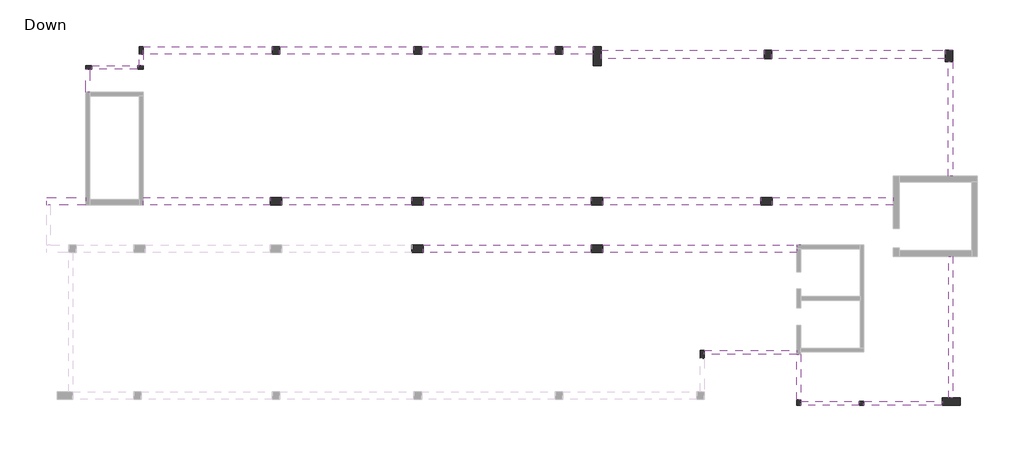
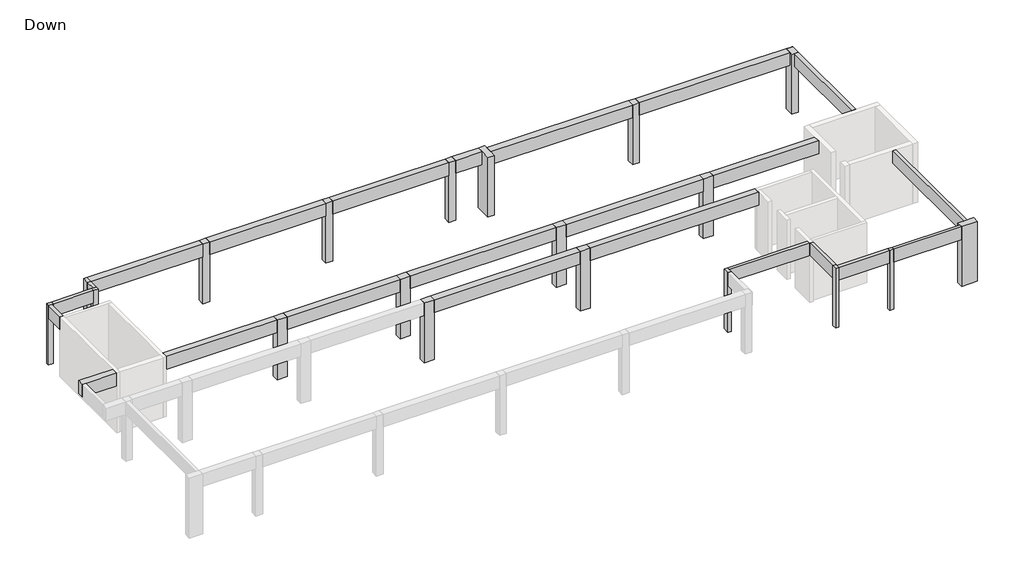
# One storey, part 2 of 2: 23 beams, 19 columns.
"""IFC4 building model written with IfcOpenShell, lengths in millimetres."""

from ifc_helpers import new_model, si_unit, frame, origin, origin_with_axes, place, context, project, spatial, polyline, outline, extrude, faceted_brep, element, save

model = new_model("IFC4")

# Units and contexts
model_context = context("Model", 3, world=origin())
ifc_project = project(units=[si_unit("LENGTHUNIT", "METRE", prefix="MILLI")], contexts=[model_context])

# Site, building, storey
site = spatial("IfcSite", under=ifc_project)
building = spatial("IfcBuilding", under=site)
storey = spatial("IfcBuildingStorey", under=building, Name="Down", Elevation=0.0)

# Beams
placement = place(None, origin())
element("IfcBeam", 1, ObjectType="Concrete Rectengular Beam : 20/80", at=placement, inside=storey, context=model_context, shape_type="Brep", body=[
    faceted_brep([(-14307.5920656, 7355.2095413, 3800.0), (-14307.5920656, 7555.2095413, 3800.0), (-16709.1027603, 7555.2095413, 3800.0), (-16709.1027603, 7355.2095413, 3800.0), (-16709.1027603, 7355.2095413, 3520.0), (-16709.1027603, 7355.2095413, 3000.0), (-14307.5920656, 7355.2095413, 3000.0), (-14307.5920656, 7355.2095413, 3520.0), (-14307.5920656, 7555.2095413, 3000.0), (-16709.1027603, 7555.2095413, 3000.0)], [[[0, 1, 2, 3]], [[0, 3, 4, 5, 6, 7]], [[8, 6, 5, 9]], [[1, 8, 9, 2]], [[1, 0, 7, 6, 8]], [[3, 2, 9, 5, 4]]]),
])
element("IfcBeam", 2, ObjectType="Concrete Rectengular Beam : 20/80", at=placement, inside=storey, context=model_context, shape_type="Brep", body=[
    faceted_brep([(-16809.1027603, 7355.2095413, 3800.0), (-17009.1027603, 7355.2095413, 3800.0), (-17009.1027603, 6157.8562202, 3800.0), (-16809.1027603, 6157.8562202, 3800.0), (-17009.1027603, 7355.2095413, 3000.0), (-17009.1027603, 6157.8562202, 3000.0), (-16809.1027603, 7355.2095413, 3000.0), (-16809.1027603, 6157.8562202, 3000.0), (-16809.1027603, 7355.2095413, 3520.0), (-16809.1027603, 6157.8562202, 3520.0)], [[[0, 1, 2, 3]], [[1, 4, 5, 2]], [[4, 6, 7, 5]], [[6, 8, 0, 3, 9, 7]], [[0, 8, 6, 4, 1]], [[3, 2, 5, 7, 9]]]),
])
element("IfcBeam", 3, ObjectType="Concrete Rectengular Beam : 20/80", at=placement, inside=storey, context=model_context, shape_type="Brep", body=[
    faceted_brep([(28136.856558, -9844.9662281, 3800.0), (28336.856558, -9844.9662281, 3800.0), (28336.856558, -2441.3717827, 3800.0), (28136.856558, -2441.3717827, 3800.0), (28336.856558, -9844.9662281, 3000.0), (28336.856558, -2441.3717827, 3000.0), (28136.856558, -9844.9662281, 3000.0), (28136.856558, -2441.3717827, 3000.0), (28136.856558, -9844.9662281, 3520.0), (28136.856558, -2441.3717827, 3520.0)], [[[0, 1, 2, 3]], [[1, 4, 5, 2]], [[4, 6, 7, 5]], [[6, 8, 0, 3, 9, 7]], [[1, 0, 8, 6, 4]], [[3, 2, 5, 7, 9]]]),
])
element("IfcBeam", 4, ObjectType="Concrete Rectengular Beam : 20/80", at=placement, inside=storey, context=model_context, shape_type="Brep", body=[
    faceted_brep([(23695.2926489, -10044.9662281, 3800.0), (23695.2926489, -10244.9662281, 3800.0), (27784.8345171, -10244.9662281, 3800.0), (27784.8345171, -10044.9662281, 3800.0), (23695.2926489, -10244.9662281, 3000.0), (27784.8345171, -10244.9662281, 3000.0), (23695.2926489, -10044.9662281, 3000.0), (27784.8345171, -10044.9662281, 3000.0), (27784.8345171, -10044.9662281, 3520.0)], [[[0, 1, 2, 3]], [[1, 4, 5, 2]], [[4, 6, 7, 5]], [[6, 0, 3, 8, 7]], [[1, 0, 6, 4]], [[3, 2, 5, 7, 8]]]),
])
element("IfcBeam", 5, ObjectType="Concrete Rectengular Beam : 20/80", at=placement, inside=storey, context=model_context, shape_type="Brep", body=[
    faceted_brep([(20395.2300261, -10044.9662281, 3800.0), (20395.2300261, -10244.9662281, 3800.0), (23445.2926489, -10244.9662281, 3800.0), (23445.2926489, -10044.9662281, 3800.0), (20395.2300261, -10044.9662281, 3000.0), (20395.2300261, -10044.9662281, 3520.0), (23445.2926489, -10044.9662281, 3000.0), (20395.2300261, -10244.9662281, 3000.0), (23445.2926489, -10244.9662281, 3000.0)], [[[0, 1, 2, 3]], [[4, 5, 0, 3, 6]], [[7, 4, 6, 8]], [[1, 7, 8, 2]], [[1, 0, 5, 4, 7]], [[3, 2, 8, 6]]]),
])
element("IfcBeam", 6, ObjectType="Concrete Rectengular Beam : 20/80", at=placement, inside=storey, context=model_context, shape_type="SweptSolid", body=[
    extrude(outline(polyline([(20195.2300261, -7584.1322554), (20395.2300261, -7584.1322554), (20395.2300261, -9947.194205), (20195.2300261, -9947.194205), (20195.2300261, -7584.1322554)])), frame((0.0, 0.0, 3000.0), z_axis=(0.0, 0.0, 1.0), x_axis=(1.0, 0.0, 0.0)), (0.0, 0.0, 1.0), 800.0),
])
element("IfcBeam", 7, ObjectType="Concrete Rectengular Beam : 20/80", at=placement, inside=storey, context=model_context, shape_type="Brep", body=[
    faceted_brep([(15344.7363769, -7371.4322554, 3800.0), (15344.7363769, -7571.4322554, 3800.0), (20195.2300261, -7571.4322554, 3800.0), (20195.2300261, -7371.4322554, 3800.0), (20195.2300261, -7371.4322554, 3520.0), (20195.2300261, -7371.4322554, 3000.0), (15344.7363769, -7371.4322554, 3000.0), (15344.7363769, -7371.4322554, 3520.0), (15344.7363769, -7571.4322554, 3000.0), (20195.2300261, -7571.4322554, 3000.0)], [[[0, 1, 2, 3]], [[0, 3, 4, 5, 6, 7]], [[8, 6, 5, 9]], [[1, 8, 9, 2]], [[1, 0, 7, 6, 8]], [[3, 2, 9, 5, 4]]]),
])
element("IfcBeam", 8, ObjectType="Concrete Rectengular Beam : 20/80", at=placement, inside=storey, context=model_context, shape_type="Brep", body=[
    faceted_brep([(-14207.5920656, 7555.2095413, 3800.0), (-14007.5920656, 7555.2095413, 3800.0), (-14007.5920656, 8151.3324092, 3800.0), (-14207.5920656, 8151.3324092, 3800.0), (-14207.5920656, 7555.2095413, 3000.0), (-14207.5920656, 8151.3324092, 3000.0), (-14007.5920656, 7555.2095413, 3000.0), (-14007.5920656, 8151.3324092, 3000.0), (-14007.5920656, 7555.2095413, 3520.0), (-14007.5920656, 8151.3324092, 3520.0)], [[[0, 1, 2, 3]], [[4, 0, 3, 5]], [[6, 4, 5, 7]], [[2, 1, 8, 6, 7, 9]], [[0, 4, 6, 8, 1]], [[5, 3, 2, 9, 7]]]),
])
element("IfcBeam", 9, ObjectType="Concrete Rectengular Beam : 25/80", at=placement, inside=storey, context=model_context, shape_type="Brep", body=[
    faceted_brep([(28351.2236194, 7751.6453791, 3800.0), (28101.2236194, 7751.6453791, 3800.0), (28101.2236194, 1758.6282173, 3800.0), (28351.2236194, 1758.6282173, 3800.0), (28101.2236194, 7751.6453791, 3520.0), (28101.2236194, 7751.6453791, 3000.0), (28101.2236194, 1758.6282173, 3000.0), (28101.2236194, 1758.6282173, 3520.0), (28351.2236194, 7751.6453791, 3000.0), (28351.2236194, 1758.6282173, 3000.0)], [[[0, 1, 2, 3]], [[1, 4, 5, 6, 7, 2]], [[5, 8, 9, 6]], [[8, 0, 3, 9]], [[1, 0, 8, 5, 4]], [[3, 2, 7, 6, 9]]]),
])
element("IfcBeam", 10, ObjectType="Concrete Rectengular Beam : 40/80", at=placement, inside=storey, context=model_context, shape_type="Brep", body=[
    faceted_brep([(-7257.9830653, 8151.3324092, 3800.0), (-7257.9830653, 8551.3324092, 3800.0), (-14007.5920656, 8551.3324092, 3800.0), (-14007.5920656, 8151.3324092, 3800.0), (-7257.9830653, 8151.3324092, 3000.0), (-14007.5920656, 8151.3324092, 3520.0), (-14007.5920656, 8151.3324092, 3000.0), (-7257.9830653, 8551.3324092, 3000.0), (-14007.5920656, 8551.3324092, 3000.0)], [[[0, 1, 2, 3]], [[4, 0, 3, 5, 6]], [[7, 4, 6, 8]], [[1, 7, 8, 2]], [[1, 0, 4, 7]], [[3, 2, 8, 6, 5]]]),
])
element("IfcBeam", 11, ObjectType="Concrete Rectengular Beam : 40/80", at=placement, inside=storey, context=model_context, shape_type="SweptSolid", body=[
    extrude(outline(polyline([(-6857.9830653, 8151.3324092), (-6857.9830653, 8551.3324092), (151.39348, 8551.3324092), (151.39348, 8151.3324092), (-6857.9830653, 8151.3324092)])), frame((0.0, 0.0, 3000.0), z_axis=(0.0, 0.0, 1.0), x_axis=(1.0, 0.0, 0.0)), (0.0, 0.0, 1.0), 800.0),
])
element("IfcBeam", 12, ObjectType="Concrete Rectengular Beam : 40/80", at=placement, inside=storey, context=model_context, shape_type="SweptSolid", body=[
    extrude(outline(polyline([(551.39348, 8151.3324092), (551.39348, 8551.3324092), (7548.8072182, 8551.3324092), (7548.8072182, 8151.3324092), (551.39348, 8151.3324092)])), frame((0.0, 0.0, 3000.0), z_axis=(0.0, 0.0, 1.0), x_axis=(1.0, 0.0, 0.0)), (0.0, 0.0, 1.0), 800.0),
])
element("IfcBeam", 13, ObjectType="Concrete Rectengular Beam : 40/80", at=placement, inside=storey, context=model_context, shape_type="Brep", body=[
    faceted_brep([(7948.8072182, 8551.3324092, 3800.0), (7948.8072182, 8151.3324092, 3800.0), (9543.2216506, 8151.3324092, 3800.0), (9543.2216506, 8551.3324092, 3800.0), (7948.8072182, 8151.3324092, 3000.0), (9543.2216506, 8151.3324092, 3000.0), (9543.2216506, 8151.3324092, 3520.0), (7948.8072182, 8551.3324092, 3000.0), (9543.2216506, 8551.3324092, 3000.0)], [[[0, 1, 2, 3]], [[1, 4, 5, 6, 2]], [[4, 7, 8, 5]], [[7, 0, 3, 8]], [[1, 0, 7, 4]], [[3, 2, 6, 5, 8]]]),
])
element("IfcBeam", 14, ObjectType="Concrete Rectengular Beam : 40/80", at=placement, inside=storey, context=model_context, shape_type="SweptSolid", body=[
    extrude(outline(polyline([(-2249.6811448, 3000.0), (-2249.6811448, 3800.0), (-1851.1339506, 3800.0), (-1851.1339506, 3520.0), (-1849.6811448, 3520.0), (-1849.6811448, 3000.0), (-2249.6811448, 3000.0)])), frame((651.39348, 0.0, 0.0), z_axis=(1.0, 0.0, 0.0), x_axis=(0.0, 1.0, 0.0)), (0.0, 0.0, 1.0), 8791.8281706),
])
element("IfcBeam", 15, ObjectType="Concrete Rectengular Beam : 40/80", at=placement, inside=storey, context=model_context, shape_type="Brep", body=[
    faceted_brep([(10043.2216506, -2249.6811448, 3800.0), (20196.3370418, -2249.6811448, 3800.0), (20196.3370418, -2051.1339506, 3800.0), (20196.3370418, -1851.1339506, 3800.0), (10043.2216506, -1851.1339506, 3800.0), (10043.2216506, -2249.6811448, 3000.0), (20196.3370418, -2249.6811448, 3000.0), (20196.3370418, -2249.6811448, 3520.0), (10043.2216506, -1849.6811448, 3000.0), (20396.3370418, -1849.6811448, 3000.0), (20396.3370418, -1851.1339506, 3000.0), (20196.3370418, -1851.1339506, 3000.0), (10043.2216506, -1849.6811448, 3520.0), (20396.3370418, -1849.6811448, 3520.0), (10043.2216506, -1851.1339506, 3520.0), (20396.3370418, -1851.1339506, 3520.0), (20196.3370418, -1851.1339506, 3520.0)], [[[0, 1, 2, 3, 4]], [[0, 5, 6, 7, 1]], [[5, 8, 9, 10, 11, 6]], [[9, 8, 12, 13]], [[5, 0, 4, 14, 12, 8]], [[11, 10, 15, 16]], [[10, 9, 13, 15]], [[1, 7, 6, 11, 16, 3, 2]], [[14, 16, 15, 13, 12]], [[16, 14, 4, 3]]]),
])
element("IfcBeam", 16, ObjectType="Concrete Rectengular Beam : 40/80", at=placement, inside=storey, context=model_context, shape_type="Brep", body=[
    faceted_brep([(-7357.9791944, 245.3255739, 3800.0), (-7357.9791944, 645.3255739, 3800.0), (-14012.0714244, 645.3255739, 3800.0), (-14012.0714244, 245.3255739, 3800.0), (-7357.9791944, 645.3255739, 3000.0), (-14012.0714244, 645.3255739, 3000.0), (-14012.0714244, 645.3255739, 3520.0), (-7357.9791944, 245.3255739, 3000.0), (-14012.0714244, 245.3255739, 3000.0)], [[[0, 1, 2, 3]], [[1, 4, 5, 6, 2]], [[4, 7, 8, 5]], [[7, 0, 3, 8]], [[1, 0, 7, 4]], [[3, 2, 6, 5, 8]]]),
])
element("IfcBeam", 17, ObjectType="Concrete Rectengular Beam : 40/80", at=placement, inside=storey, context=model_context, shape_type="SweptSolid", body=[
    extrude(outline(polyline([(51.396575, 645.3255739), (51.396575, 245.3255739), (-6757.9791944, 245.3255739), (-6757.9791944, 645.3255739), (51.396575, 645.3255739)])), frame((0.0, 0.0, 3000.0), z_axis=(0.0, 0.0, 1.0), x_axis=(1.0, 0.0, 0.0)), (0.0, 0.0, 1.0), 800.0),
])
element("IfcBeam", 18, ObjectType="Concrete Rectengular Beam : 40/80", at=placement, inside=storey, context=model_context, shape_type="SweptSolid", body=[
    extrude(outline(polyline([(9443.2258738, 645.3255739), (9443.2258738, 245.3255739), (651.396575, 245.3255739), (651.396575, 645.3255739), (9443.2258738, 645.3255739)])), frame((0.0, 0.0, 3000.0), z_axis=(0.0, 0.0, 1.0), x_axis=(1.0, 0.0, 0.0)), (0.0, 0.0, 1.0), 800.0),
])
element("IfcBeam", 19, ObjectType="Concrete Rectengular Beam : 40/80", at=placement, inside=storey, context=model_context, shape_type="SweptSolid", body=[
    extrude(outline(polyline([(18292.1885308, 645.3255739), (18292.1885308, 245.3255739), (10043.2258738, 245.3255739), (10043.2258738, 645.3255739), (18292.1885308, 645.3255739)])), frame((0.0, 0.0, 3000.0), z_axis=(0.0, 0.0, 1.0), x_axis=(1.0, 0.0, 0.0)), (0.0, 0.0, 1.0), 800.0),
])
element("IfcBeam", 20, ObjectType="Concrete Rectengular Beam : 40/80", at=placement, inside=storey, context=model_context, shape_type="Brep", body=[
    faceted_brep([(18892.1885308, 645.3255739, 3800.0), (18892.1885308, 245.3255739, 3800.0), (25241.4195047, 245.3255739, 3800.0), (25241.4195047, 645.3255739, 3800.0), (18892.1885308, 245.3255739, 3000.0), (25241.4195047, 245.3255739, 3000.0), (25241.4195047, 245.3255739, 3520.0), (18892.1885308, 645.3255739, 3000.0), (25241.4195047, 645.3255739, 3000.0), (25241.4195047, 645.3255739, 3520.0)], [[[0, 1, 2, 3]], [[1, 4, 5, 6, 2]], [[4, 7, 8, 5]], [[7, 0, 3, 9, 8]], [[1, 0, 7, 4]], [[3, 2, 6, 5, 8, 9]]]),
])
element("IfcBeam", 21, ObjectType="Concrete Rectengular Beam : 40/80", at=placement, inside=storey, context=model_context, shape_type="Brep", body=[
    faceted_brep([(-19067.5920656, 645.3255739, 3800.0), (-19067.5920656, 245.3255739, 3800.0), (-18867.5920656, 245.3255739, 3800.0), (-17009.1027603, 245.3255739, 3800.0), (-17009.1027603, 645.3255739, 3800.0), (-19067.5920656, 645.3255739, 3000.0), (-17009.1027603, 645.3255739, 3000.0), (-19067.5920656, 245.3255739, 3000.0), (-17009.1027603, 245.3255739, 3000.0), (-18867.5920656, 245.3255739, 3000.0)], [[[0, 1, 2, 3, 4]], [[5, 0, 4, 6]], [[7, 5, 6, 8, 9]], [[1, 7, 9, 8, 3, 2]], [[1, 0, 5, 7]], [[4, 3, 8, 6]]]),
])
element("IfcBeam", 22, ObjectType="Concrete Rectengular Beam : 43/80", at=placement, inside=storey, context=model_context, shape_type="Brep", body=[
    faceted_brep([(18471.5975134, 7925.3792217, 3800.0), (18471.5975134, 8355.3792217, 3800.0), (9943.2216506, 8355.3792217, 3800.0), (9943.2216506, 7925.3792217, 3800.0), (18471.5975134, 8355.3792217, 3000.0), (9943.2216506, 8355.3792217, 3000.0), (9943.2216506, 8355.3792217, 3520.0), (18471.5975134, 7925.3792217, 3000.0), (9943.2216506, 7925.3792217, 3000.0), (9943.2216506, 7925.3792217, 3520.0), (18471.5975134, 7925.3792217, 3520.0)], [[[0, 1, 2, 3]], [[1, 4, 5, 6, 2]], [[4, 7, 8, 5]], [[0, 3, 9, 8, 7, 10]], [[1, 0, 10, 7, 4]], [[3, 2, 6, 5, 8, 9]]]),
])
element("IfcBeam", 23, ObjectType="Concrete Rectengular Beam : 43/80", at=placement, inside=storey, context=model_context, shape_type="Brep", body=[
    faceted_brep([(18871.5975134, 8355.3792217, 3800.0), (18871.5975134, 7925.3792217, 3800.0), (27951.2236194, 7925.3792217, 3800.0), (27951.2236194, 8351.6453791, 3800.0), (28351.2236194, 8351.6453791, 3800.0), (28351.2236194, 8355.3792217, 3800.0), (26203.2216506, 8355.3792217, 3800.0), (18871.5975134, 7925.3792217, 3520.0), (18871.5975134, 7925.3792217, 3000.0), (27951.2236194, 7925.3792217, 3000.0), (27951.2236194, 7925.3792217, 3520.0), (18871.5975134, 8355.3792217, 3000.0), (28351.2236194, 8355.3792217, 3000.0), (28351.2236194, 8351.6453791, 3000.0), (27951.2236194, 8351.6453791, 3000.0)], [[[0, 1, 2, 3, 4, 5, 6]], [[2, 1, 7, 8, 9, 10]], [[8, 11, 12, 13, 14, 9]], [[11, 0, 6, 5, 12]], [[1, 0, 11, 8, 7]], [[14, 3, 2, 10, 9]], [[3, 14, 13, 4]], [[12, 5, 4, 13]]]),
])

# Columns
element("IfcColumn", 24, ObjectType="Concrete Rectengular Column : 20/25", at=placement, inside=storey, context=model_context, shape_type="SweptSolid", body=[
    extrude(outline(polyline([(23445.2926489, -10044.9662281), (23695.2926489, -10044.9662281), (23695.2926489, -10244.9662281), (23445.2926489, -10244.9662281), (23445.2926489, -10044.9662281)])), origin_with_axes(), (0.0, 0.0, 1.0), 3800.0),
])
element("IfcColumn", 25, ObjectType="Concrete Rectengular Column : 20/30", at=placement, inside=storey, context=model_context, shape_type="Brep", body=[
    faceted_brep([(20395.2300261, -9947.194205, 0.0), (20395.2300261, -10247.194205, 0.0), (20195.2300261, -10247.194205, 0.0), (20195.2300261, -9947.194205, 0.0), (20395.2300261, -9947.194205, 3800.0), (20395.2300261, -10044.9662281, 3800.0), (20395.2300261, -10247.194205, 3800.0), (20195.2300261, -10247.194205, 3800.0), (20195.2300261, -9947.194205, 3800.0)], [[[0, 1, 2, 3]], [[4, 5, 6, 1, 0]], [[6, 7, 2, 1]], [[7, 8, 3, 2]], [[8, 4, 0, 3]], [[4, 8, 7, 6, 5]]]),
])
element("IfcColumn", 26, ObjectType="Concrete Rectengular Column : 20/30", at=placement, inside=storey, context=model_context, shape_type="Brep", body=[
    faceted_brep([(-14307.5920656, 7555.2095413, 0.0), (-14007.5920656, 7555.2095413, 0.0), (-14007.5920656, 7355.2095413, 0.0), (-14307.5920656, 7355.2095413, 0.0), (-14307.5920656, 7555.2095413, 3800.0), (-14007.5920656, 7555.2095413, 3800.0), (-14007.5920656, 7355.2095413, 3800.0), (-14007.5920656, 7355.2095413, 3520.0), (-14307.5920656, 7355.2095413, 3800.0)], [[[0, 1, 2, 3]], [[4, 5, 1, 0]], [[5, 6, 7, 2, 1]], [[6, 8, 3, 2, 7]], [[8, 4, 0, 3]], [[4, 8, 6, 5]]]),
])
element("IfcColumn", 27, ObjectType="Concrete Rectengular Column : 20/30", at=placement, inside=storey, context=model_context, shape_type="Brep", body=[
    faceted_brep([(-17009.1027603, 7555.2095413, 0.0), (-16709.1027603, 7555.2095413, 0.0), (-16709.1027603, 7355.2095413, 0.0), (-17009.1027603, 7355.2095413, 0.0), (-17009.1027603, 7555.2095413, 3800.0), (-16709.1027603, 7555.2095413, 3800.0), (-16709.1027603, 7355.2095413, 3800.0), (-16809.1027603, 7355.2095413, 3800.0), (-17009.1027603, 7355.2095413, 3800.0)], [[[0, 1, 2, 3]], [[4, 5, 1, 0]], [[5, 6, 2, 1]], [[6, 7, 8, 3, 2]], [[8, 4, 0, 3]], [[4, 8, 7, 6, 5]]]),
])
element("IfcColumn", 28, ObjectType="Concrete Rectengular Column : 20/40", at=placement, inside=storey, context=model_context, shape_type="Brep", body=[
    faceted_brep([(15344.7363769, -7371.4322554, 0.0), (15344.7363769, -7771.4322554, 0.0), (15144.7363769, -7771.4322554, 0.0), (15144.7363769, -7371.4322554, 0.0), (15344.7363769, -7371.4322554, 3800.0), (15344.7363769, -7771.4322554, 3800.0), (15144.7363769, -7771.4322554, 3800.0), (15144.7363769, -7371.4322554, 3800.0), (15144.7363769, -7371.4322554, 3520.0)], [[[0, 1, 2, 3]], [[4, 5, 1, 0]], [[5, 6, 2, 1]], [[6, 7, 8, 3, 2]], [[7, 4, 0, 3, 8]], [[4, 7, 6, 5]]]),
])
element("IfcColumn", 29, ObjectType="Concrete Rectengular Column : 20/40", at=placement, inside=storey, context=model_context, shape_type="SweptSolid", body=[
    extrude(outline(polyline([(-14007.5920656, 8551.3324092), (-14007.5920656, 8151.3324092), (-14207.5920656, 8151.3324092), (-14207.5920656, 8551.3324092), (-14007.5920656, 8551.3324092)])), origin_with_axes(), (0.0, 0.0, 1.0), 3800.0),
])
element("IfcColumn", 30, ObjectType="Concrete Rectengular Column : 40/100", at=placement, inside=storey, context=model_context, shape_type="Brep", body=[
    faceted_brep([(9943.2216506, 8551.6453791, 0.0), (9943.2216506, 7551.6453791, 0.0), (9543.2216506, 7551.6453791, 0.0), (9543.2216506, 8551.6453791, 0.0), (9943.2216506, 8551.6453791, 3800.0), (9943.2216506, 8355.3792217, 3800.0), (9943.2216506, 7925.3792217, 3800.0), (9943.2216506, 7551.6453791, 3800.0), (9943.2216506, 7551.6453791, 3520.0), (9543.2216506, 7551.6453791, 3800.0), (9543.2216506, 7551.6453791, 3520.0), (9543.2216506, 8151.3324092, 3800.0), (9543.2216506, 8551.6453791, 3800.0)], [[[0, 1, 2, 3]], [[4, 5, 6, 7, 8, 1, 0]], [[7, 9, 10, 2, 1, 8]], [[9, 11, 12, 3, 2, 10]], [[12, 4, 0, 3]], [[4, 12, 11, 9, 7, 6, 5]]]),
])
element("IfcColumn", 31, ObjectType="Concrete Rectengular Column : 40/40", at=placement, inside=storey, context=model_context, shape_type="SweptSolid", body=[
    extrude(outline(polyline([(-6857.9830653, 8551.3324092), (-6857.9830653, 8151.3324092), (-7257.9830653, 8151.3324092), (-7257.9830653, 8551.3324092), (-6857.9830653, 8551.3324092)])), origin_with_axes(), (0.0, 0.0, 1.0), 3800.0),
])
element("IfcColumn", 32, ObjectType="Concrete Rectengular Column : 40/40", at=placement, inside=storey, context=model_context, shape_type="SweptSolid", body=[
    extrude(outline(polyline([(551.39348, 8551.3324092), (551.39348, 8151.3324092), (151.39348, 8151.3324092), (151.39348, 8551.3324092), (551.39348, 8551.3324092)])), origin_with_axes(), (0.0, 0.0, 1.0), 3800.0),
])
element("IfcColumn", 33, ObjectType="Concrete Rectengular Column : 40/40", at=placement, inside=storey, context=model_context, shape_type="SweptSolid", body=[
    extrude(outline(polyline([(7948.8072182, 8551.3324092), (7948.8072182, 8151.3324092), (7548.8072182, 8151.3324092), (7548.8072182, 8551.3324092), (7948.8072182, 8551.3324092)])), origin_with_axes(), (0.0, 0.0, 1.0), 3800.0),
])
element("IfcColumn", 34, ObjectType="Concrete Rectengular Column : 40/43", at=placement, inside=storey, context=model_context, shape_type="SweptSolid", body=[
    extrude(outline(polyline([(18871.5975134, 8355.3792217), (18871.5975134, 7925.3792217), (18471.5975134, 7925.3792217), (18471.5975134, 8355.3792217), (18871.5975134, 8355.3792217)])), origin_with_axes(), (0.0, 0.0, 1.0), 3800.0),
])
element("IfcColumn", 35, ObjectType="Concrete Rectengular Column : 40/60", at=placement, inside=storey, context=model_context, shape_type="Brep", body=[
    faceted_brep([(9443.2216506, -1849.6811448, 0.0), (10043.2216506, -1849.6811448, 0.0), (10043.2216506, -2249.6811448, 0.0), (9443.2216506, -2249.6811448, 0.0), (9443.2216506, -1849.6811448, 3800.0), (10043.2216506, -1849.6811448, 3800.0), (10043.2216506, -1849.6811448, 3520.0), (9443.2216506, -1849.6811448, 3520.0), (10043.2216506, -1851.1339506, 3800.0), (10043.2216506, -2249.6811448, 3800.0), (9443.2216506, -2249.6811448, 3800.0), (9443.2216506, -1851.1339506, 3800.0)], [[[0, 1, 2, 3]], [[4, 5, 6, 1, 0, 7]], [[5, 8, 9, 2, 1, 6]], [[9, 10, 3, 2]], [[10, 11, 4, 7, 0, 3]], [[4, 11, 10, 9, 8, 5]]]),
])
element("IfcColumn", 36, ObjectType="Concrete Rectengular Column : 40/60", at=placement, inside=storey, context=model_context, shape_type="Brep", body=[
    faceted_brep([(51.39348, -1849.6811448, 0.0), (651.39348, -1849.6811448, 0.0), (651.39348, -2249.6811448, 0.0), (51.39348, -2249.6811448, 0.0), (51.39348, -1849.6811448, 3800.0), (651.39348, -1849.6811448, 3800.0), (651.39348, -1849.6811448, 3520.0), (51.39348, -1849.6811448, 3520.0), (651.39348, -1851.1339506, 3800.0), (651.39348, -2249.6811448, 3800.0), (51.39348, -2249.6811448, 3800.0), (51.39348, -1851.1339506, 3800.0)], [[[0, 1, 2, 3]], [[4, 5, 6, 1, 0, 7]], [[5, 8, 9, 2, 1, 6]], [[9, 10, 3, 2]], [[10, 11, 4, 7, 0, 3]], [[4, 11, 10, 9, 8, 5]]]),
])
element("IfcColumn", 37, ObjectType="Concrete Rectengular Column : 40/60", at=placement, inside=storey, context=model_context, shape_type="SweptSolid", body=[
    extrude(outline(polyline([(18292.1885308, 645.3255739), (18892.1885308, 645.3255739), (18892.1885308, 245.3255739), (18292.1885308, 245.3255739), (18292.1885308, 645.3255739)])), origin_with_axes(), (0.0, 0.0, 1.0), 3800.0),
])
element("IfcColumn", 38, ObjectType="Concrete Rectengular Column : 40/60", at=placement, inside=storey, context=model_context, shape_type="SweptSolid", body=[
    extrude(outline(polyline([(9443.2258738, 645.3255739), (10043.2258738, 645.3255739), (10043.2258738, 245.3255739), (9443.2258738, 245.3255739), (9443.2258738, 645.3255739)])), origin_with_axes(), (0.0, 0.0, 1.0), 3800.0),
])
element("IfcColumn", 39, ObjectType="Concrete Rectengular Column : 40/60", at=placement, inside=storey, context=model_context, shape_type="SweptSolid", body=[
    extrude(outline(polyline([(51.396575, 645.3255739), (651.396575, 645.3255739), (651.396575, 245.3255739), (51.396575, 245.3255739), (51.396575, 645.3255739)])), origin_with_axes(), (0.0, 0.0, 1.0), 3800.0),
])
element("IfcColumn", 40, ObjectType="Concrete Rectengular Column : 40/60", at=placement, inside=storey, context=model_context, shape_type="SweptSolid", body=[
    extrude(outline(polyline([(-7357.9791944, 645.3255739), (-6757.9791944, 645.3255739), (-6757.9791944, 245.3255739), (-7357.9791944, 245.3255739), (-7357.9791944, 645.3255739)])), origin_with_axes(), (0.0, 0.0, 1.0), 3800.0),
])
element("IfcColumn", 41, ObjectType="Concrete Rectengular Column : 40/60", at=placement, inside=storey, context=model_context, shape_type="Brep", body=[
    faceted_brep([(28351.2236194, 8351.6453791, 0.0), (28351.2236194, 7751.6453791, 0.0), (27951.2236194, 7751.6453791, 0.0), (27951.2236194, 8351.6453791, 0.0), (28351.2236194, 8351.6453791, 3800.0), (28351.2236194, 7751.6453791, 3800.0), (28101.2236194, 7751.6453791, 3800.0), (27951.2236194, 7751.6453791, 3800.0), (27951.2236194, 7751.6453791, 3520.0), (27951.2236194, 7925.3792217, 3800.0), (27951.2236194, 8351.6453791, 3800.0)], [[[0, 1, 2, 3]], [[4, 5, 1, 0]], [[5, 6, 7, 8, 2, 1]], [[7, 9, 10, 3, 2, 8]], [[10, 4, 0, 3]], [[4, 10, 9, 7, 6, 5]]]),
])
element("IfcColumn", 42, ObjectType="Concrete Rectengular Column : 40/95", at=placement, inside=storey, context=model_context, shape_type="Brep", body=[
    faceted_brep([(27784.8345171, -9844.9662281, 0.0), (28734.8345171, -9844.9662281, 0.0), (28734.8345171, -10244.9662281, 0.0), (27784.8345171, -10244.9662281, 0.0), (27784.8345171, -9844.9662281, 3800.0), (28136.856558, -9844.9662281, 3800.0), (28734.8345171, -9844.9662281, 3800.0), (27784.8345171, -9844.9662281, 3520.0), (28734.8345171, -10244.9662281, 3800.0), (27784.8345171, -10244.9662281, 3800.0), (27784.8345171, -10044.9662281, 3800.0)], [[[0, 1, 2, 3]], [[4, 5, 6, 1, 0, 7]], [[6, 8, 2, 1]], [[8, 9, 3, 2]], [[9, 10, 4, 7, 0, 3]], [[4, 10, 9, 8, 6, 5]]]),
])

save(model, "model.ifc")

# Revit data of these elements
# Type "Concrete Rectengular Beam : 20/80"
#   Length [instance default] = 152.4 cm
#   b = 20 cm
#   h = 80 cm
#   Structural Material [instance default] = Concrete
#   Assembly Code = ""
# Type "Concrete Rectengular Beam : 25/80"
#   Length [instance default] = 152.4 cm
#   b = 25 cm
#   h = 80 cm
#   Structural Material [instance default] = Concrete
#   Assembly Code = ""
# Type "Concrete Rectengular Beam : 40/80"
#   Length [instance default] = 152.4 cm
#   b = 40 cm
#   h = 80 cm
#   Structural Material [instance default] = Concrete
#   Assembly Code = ""
# Type "Concrete Rectengular Beam : 43/80"
#   Length [instance default] = 152.4 cm
#   b = 43 cm
#   h = 80 cm
#   Structural Material [instance default] = Concrete
#   Assembly Code = ""
# Type "Concrete Rectengular Column : 20/25"
#   b = 20 cm
#   h = 25 cm
#   Structural Material [instance default] = Concrete
# Type "Concrete Rectengular Column : 20/30"
#   b = 20 cm
#   h = 30 cm
#   Structural Material [instance default] = Concrete
# Type "Concrete Rectengular Column : 20/40"
#   b = 20 cm
#   h = 40 cm
#   Structural Material [instance default] = Concrete
# Type "Concrete Rectengular Column : 40/100"
#   b = 40 cm
#   h = 100 cm
#   Structural Material [instance default] = Concrete
# Type "Concrete Rectengular Column : 40/40"
#   b = 40 cm
#   h = 40 cm
#   Structural Material [instance default] = Concrete
# Type "Concrete Rectengular Column : 40/43"
#   b = 40 cm
#   h = 43 cm
#   Structural Material [instance default] = Concrete
# Type "Concrete Rectengular Column : 40/60"
#   b = 40 cm
#   h = 60 cm
#   Structural Material [instance default] = Concrete
# Type "Concrete Rectengular Column : 40/95"
#   b = 40 cm
#   h = 95 cm
#   Structural Material [instance default] = Concrete
# Element 1 (IfcBeam, "Concrete Rectengular Beam : 20/80")
#   Comments = ""
#   Mark = "B1"
#   SOFiSTiK_AMG_Comments = ""
#   SOFiSTiK_AMG_Scheduled = yes
#   SOFiSTiK_AMG_Adjusted = yes
#   Structural Material = Concrete
#   Phase Created = New Construction
#   Materials on its faces: "Concrete"
# Element 2 (IfcBeam, "Concrete Rectengular Beam : 20/80")
#   Comments = ""
#   Mark = "B2"
#   SOFiSTiK_AMG_Comments = ""
#   SOFiSTiK_AMG_Scheduled = yes
#   SOFiSTiK_AMG_Adjusted = yes
#   Structural Material = Concrete
#   Phase Created = New Construction
#   Materials on its faces: "Concrete"
# Element 3 (IfcBeam, "Concrete Rectengular Beam : 20/80")
#   Comments = ""
#   Mark = "B3"
#   SOFiSTiK_AMG_Comments = ""
#   SOFiSTiK_AMG_Scheduled = yes
#   SOFiSTiK_AMG_Adjusted = yes
#   Structural Material = Concrete
#   Phase Created = New Construction
#   Materials on its faces: "Concrete"
# Element 4 (IfcBeam, "Concrete Rectengular Beam : 20/80")
#   Comments = ""
#   Mark = "B4"
#   SOFiSTiK_AMG_Comments = ""
#   SOFiSTiK_AMG_Scheduled = yes
#   SOFiSTiK_AMG_Adjusted = yes
#   Structural Material = Concrete
#   Phase Created = New Construction
#   Materials on its faces: "Concrete"
# Element 5 (IfcBeam, "Concrete Rectengular Beam : 20/80")
#   Comments = ""
#   Mark = "B5"
#   SOFiSTiK_AMG_Comments = ""
#   SOFiSTiK_AMG_Scheduled = yes
#   SOFiSTiK_AMG_Adjusted = yes
#   Structural Material = Concrete
#   Phase Created = New Construction
#   Materials on its faces: "Concrete"
# Element 6 (IfcBeam, "Concrete Rectengular Beam : 20/80")
#   Comments = ""
#   Mark = "B6"
#   SOFiSTiK_AMG_Comments = ""
#   SOFiSTiK_AMG_Scheduled = yes
#   SOFiSTiK_AMG_Adjusted = yes
#   Structural Material = Concrete
#   Phase Created = New Construction
#   Materials on its faces: "Concrete"
# Element 7 (IfcBeam, "Concrete Rectengular Beam : 20/80")
#   Comments = ""
#   Mark = "B7"
#   SOFiSTiK_AMG_Comments = ""
#   SOFiSTiK_AMG_Scheduled = yes
#   SOFiSTiK_AMG_Adjusted = yes
#   Structural Material = Concrete
#   Phase Created = New Construction
#   Materials on its faces: "Concrete"
# Element 8 (IfcBeam, "Concrete Rectengular Beam : 20/80")
#   Comments = ""
#   Mark = "B11"
#   SOFiSTiK_AMG_Comments = ""
#   SOFiSTiK_AMG_Scheduled = yes
#   SOFiSTiK_AMG_Adjusted = yes
#   Structural Material = Concrete
#   Phase Created = New Construction
#   Materials on its faces: "Concrete"
# Element 9 (IfcBeam, "Concrete Rectengular Beam : 25/80")
#   Comments = ""
#   Mark = "B12"
#   SOFiSTiK_AMG_Comments = ""
#   SOFiSTiK_AMG_Scheduled = yes
#   SOFiSTiK_AMG_Adjusted = yes
#   Structural Material = Concrete
#   Phase Created = New Construction
#   Materials on its faces: "Concrete"
# Element 10 (IfcBeam, "Concrete Rectengular Beam : 40/80")
#   Comments = ""
#   Mark = "B13"
#   SOFiSTiK_AMG_Comments = ""
#   SOFiSTiK_AMG_Scheduled = yes
#   SOFiSTiK_AMG_Adjusted = yes
#   Structural Material = Concrete
#   Phase Created = New Construction
#   Materials on its faces: "Concrete"
# Element 11 (IfcBeam, "Concrete Rectengular Beam : 40/80")
#   Comments = ""
#   Mark = "B14"
#   SOFiSTiK_AMG_Comments = ""
#   SOFiSTiK_AMG_Scheduled = yes
#   SOFiSTiK_AMG_Adjusted = yes
#   Structural Material = Concrete
#   Phase Created = New Construction
#   Materials on its faces: "Concrete"
# Element 12 (IfcBeam, "Concrete Rectengular Beam : 40/80")
#   Comments = ""
#   Mark = "B15"
#   SOFiSTiK_AMG_Comments = ""
#   SOFiSTiK_AMG_Scheduled = yes
#   SOFiSTiK_AMG_Adjusted = yes
#   Structural Material = Concrete
#   Phase Created = New Construction
#   Materials on its faces: "Concrete"
# Element 13 (IfcBeam, "Concrete Rectengular Beam : 40/80")
#   Comments = ""
#   Mark = "B16"
#   SOFiSTiK_AMG_Comments = ""
#   SOFiSTiK_AMG_Scheduled = yes
#   SOFiSTiK_AMG_Adjusted = yes
#   Structural Material = Concrete
#   Phase Created = New Construction
#   Materials on its faces: "Concrete"
# Element 14 (IfcBeam, "Concrete Rectengular Beam : 40/80")
#   Comments = ""
#   Mark = "B25"
#   SOFiSTiK_AMG_Comments = ""
#   SOFiSTiK_AMG_Scheduled = yes
#   SOFiSTiK_AMG_Adjusted = yes
#   Structural Material = Concrete
#   Phase Created = New Construction
#   Materials on its faces: "Concrete"
# Element 15 (IfcBeam, "Concrete Rectengular Beam : 40/80")
#   Comments = ""
#   Mark = "B26"
#   SOFiSTiK_AMG_Comments = ""
#   SOFiSTiK_AMG_Scheduled = yes
#   SOFiSTiK_AMG_Adjusted = yes
#   Structural Material = Concrete
#   Phase Created = New Construction
#   Materials on its faces: "Concrete"
# Element 16 (IfcBeam, "Concrete Rectengular Beam : 40/80")
#   Comments = ""
#   Mark = "B27"
#   SOFiSTiK_AMG_Comments = ""
#   SOFiSTiK_AMG_Scheduled = yes
#   SOFiSTiK_AMG_Adjusted = yes
#   Structural Material = Concrete
#   Phase Created = New Construction
#   Materials on its faces: "Concrete"
# Element 17 (IfcBeam, "Concrete Rectengular Beam : 40/80")
#   Comments = ""
#   Mark = "B28"
#   SOFiSTiK_AMG_Comments = ""
#   SOFiSTiK_AMG_Scheduled = yes
#   SOFiSTiK_AMG_Adjusted = yes
#   Structural Material = Concrete
#   Phase Created = New Construction
#   Materials on its faces: "Concrete"
# Element 18 (IfcBeam, "Concrete Rectengular Beam : 40/80")
#   Comments = ""
#   Mark = "B29"
#   SOFiSTiK_AMG_Comments = ""
#   SOFiSTiK_AMG_Scheduled = yes
#   SOFiSTiK_AMG_Adjusted = yes
#   Structural Material = Concrete
#   Phase Created = New Construction
#   Materials on its faces: "Concrete"
# Element 19 (IfcBeam, "Concrete Rectengular Beam : 40/80")
#   Comments = ""
#   Mark = "B30"
#   SOFiSTiK_AMG_Comments = ""
#   SOFiSTiK_AMG_Scheduled = yes
#   SOFiSTiK_AMG_Adjusted = yes
#   Structural Material = Concrete
#   Phase Created = New Construction
#   Materials on its faces: "Concrete"
# Element 20 (IfcBeam, "Concrete Rectengular Beam : 40/80")
#   Comments = ""
#   Mark = "B31"
#   SOFiSTiK_AMG_Comments = ""
#   SOFiSTiK_AMG_Scheduled = yes
#   SOFiSTiK_AMG_Adjusted = yes
#   Structural Material = Concrete
#   Phase Created = New Construction
#   Materials on its faces: "Concrete"
# Element 21 (IfcBeam, "Concrete Rectengular Beam : 40/80")
#   Comments = ""
#   Mark = "B32"
#   SOFiSTiK_AMG_Comments = ""
#   SOFiSTiK_AMG_Scheduled = yes
#   SOFiSTiK_AMG_Adjusted = yes
#   Structural Material = Concrete
#   Phase Created = New Construction
#   Materials on its faces: "Concrete"
# Element 22 (IfcBeam, "Concrete Rectengular Beam : 43/80")
#   Comments = ""
#   Mark = "B34"
#   SOFiSTiK_AMG_Comments = ""
#   SOFiSTiK_AMG_Scheduled = yes
#   SOFiSTiK_AMG_Adjusted = yes
#   Structural Material = Concrete
#   Phase Created = New Construction
#   Materials on its faces: "Concrete"
# Element 23 (IfcBeam, "Concrete Rectengular Beam : 43/80")
#   Comments = ""
#   Mark = "B35"
#   SOFiSTiK_AMG_Comments = ""
#   SOFiSTiK_AMG_Scheduled = yes
#   SOFiSTiK_AMG_Adjusted = yes
#   Structural Material = Concrete
#   Phase Created = New Construction
#   Materials on its faces: "Concrete"
# Element 24 (IfcColumn, "Concrete Rectengular Column : 20/25")
#   Comments = ""
#   Mark = "C1"
#   SOFiSTiK_AMG_Comments = ""
#   SOFiSTiK_AMG_Scheduled = yes
#   SOFiSTiK_AMG_Adjusted = yes
#   Structural Material = Concrete
#   Phase Created = New Construction
#   Materials on its faces: "Concrete"
# Element 25 (IfcColumn, "Concrete Rectengular Column : 20/30")
#   Comments = ""
#   Mark = "C2"
#   SOFiSTiK_AMG_Comments = ""
#   SOFiSTiK_AMG_Scheduled = yes
#   SOFiSTiK_AMG_Adjusted = yes
#   Structural Material = Concrete
#   Phase Created = New Construction
#   Materials on its faces: "Concrete"
# Element 26 (IfcColumn, "Concrete Rectengular Column : 20/30")
#   Comments = ""
#   Mark = "C3"
#   SOFiSTiK_AMG_Comments = ""
#   SOFiSTiK_AMG_Scheduled = yes
#   SOFiSTiK_AMG_Adjusted = yes
#   Structural Material = Concrete
#   Phase Created = New Construction
#   Materials on its faces: "Concrete"
# Element 27 (IfcColumn, "Concrete Rectengular Column : 20/30")
#   Comments = ""
#   Mark = "C4"
#   SOFiSTiK_AMG_Comments = ""
#   SOFiSTiK_AMG_Scheduled = yes
#   SOFiSTiK_AMG_Adjusted = yes
#   Structural Material = Concrete
#   Phase Created = New Construction
#   Materials on its faces: "Concrete"
# Element 28 (IfcColumn, "Concrete Rectengular Column : 20/40")
#   Comments = ""
#   Mark = "C5"
#   SOFiSTiK_AMG_Comments = ""
#   SOFiSTiK_AMG_Scheduled = yes
#   SOFiSTiK_AMG_Adjusted = yes
#   Structural Material = Concrete
#   Phase Created = New Construction
#   Materials on its faces: "Concrete"
# Element 29 (IfcColumn, "Concrete Rectengular Column : 20/40")
#   Comments = ""
#   Mark = "C6"
#   SOFiSTiK_AMG_Comments = ""
#   SOFiSTiK_AMG_Scheduled = yes
#   SOFiSTiK_AMG_Adjusted = yes
#   Structural Material = Concrete
#   Phase Created = New Construction
#   Materials on its faces: "Concrete"
# Element 30 (IfcColumn, "Concrete Rectengular Column : 40/100")
#   Comments = ""
#   Mark = "C7"
#   SOFiSTiK_AMG_Comments = ""
#   SOFiSTiK_AMG_Scheduled = yes
#   SOFiSTiK_AMG_Adjusted = yes
#   Structural Material = Concrete
#   Phase Created = New Construction
#   Materials on its faces: "Concrete"
# Element 31 (IfcColumn, "Concrete Rectengular Column : 40/40")
#   Comments = ""
#   Mark = "C14"
#   SOFiSTiK_AMG_Comments = ""
#   SOFiSTiK_AMG_Scheduled = yes
#   SOFiSTiK_AMG_Adjusted = yes
#   Structural Material = Concrete
#   Phase Created = New Construction
#   Materials on its faces: "Concrete"
# Element 32 (IfcColumn, "Concrete Rectengular Column : 40/40")
#   Comments = ""
#   Mark = "C15"
#   SOFiSTiK_AMG_Comments = ""
#   SOFiSTiK_AMG_Scheduled = yes
#   SOFiSTiK_AMG_Adjusted = yes
#   Structural Material = Concrete
#   Phase Created = New Construction
#   Materials on its faces: "Concrete"
# Element 33 (IfcColumn, "Concrete Rectengular Column : 40/40")
#   Comments = ""
#   Mark = "C16"
#   SOFiSTiK_AMG_Comments = ""
#   SOFiSTiK_AMG_Scheduled = yes
#   SOFiSTiK_AMG_Adjusted = yes
#   Structural Material = Concrete
#   Phase Created = New Construction
#   Materials on its faces: "Concrete"
# Element 34 (IfcColumn, "Concrete Rectengular Column : 40/43")
#   Comments = ""
#   Mark = "C17"
#   SOFiSTiK_AMG_Comments = ""
#   SOFiSTiK_AMG_Scheduled = yes
#   SOFiSTiK_AMG_Adjusted = yes
#   Structural Material = Concrete
#   Phase Created = New Construction
#   Materials on its faces: "Concrete"
# Element 35 (IfcColumn, "Concrete Rectengular Column : 40/60")
#   Comments = ""
#   Mark = "C20"
#   SOFiSTiK_AMG_Comments = ""
#   SOFiSTiK_AMG_Scheduled = yes
#   SOFiSTiK_AMG_Adjusted = yes
#   Structural Material = Concrete
#   Phase Created = New Construction
#   Materials on its faces: "Concrete"
# Element 36 (IfcColumn, "Concrete Rectengular Column : 40/60")
#   Comments = ""
#   Mark = "C21"
#   SOFiSTiK_AMG_Comments = ""
#   SOFiSTiK_AMG_Scheduled = yes
#   SOFiSTiK_AMG_Adjusted = yes
#   Structural Material = Concrete
#   Phase Created = New Construction
#   Materials on its faces: "Concrete"
# Element 37 (IfcColumn, "Concrete Rectengular Column : 40/60")
#   Comments = ""
#   Mark = "C22"
#   SOFiSTiK_AMG_Comments = ""
#   SOFiSTiK_AMG_Scheduled = yes
#   SOFiSTiK_AMG_Adjusted = yes
#   Structural Material = Concrete
#   Phase Created = New Construction
#   Materials on its faces: "Concrete"
# Element 38 (IfcColumn, "Concrete Rectengular Column : 40/60")
#   Comments = ""
#   Mark = "C23"
#   SOFiSTiK_AMG_Comments = ""
#   SOFiSTiK_AMG_Scheduled = yes
#   SOFiSTiK_AMG_Adjusted = yes
#   Structural Material = Concrete
#   Phase Created = New Construction
#   Materials on its faces: "Concrete"
# Element 39 (IfcColumn, "Concrete Rectengular Column : 40/60")
#   Comments = ""
#   Mark = "C24"
#   SOFiSTiK_AMG_Comments = ""
#   SOFiSTiK_AMG_Scheduled = yes
#   SOFiSTiK_AMG_Adjusted = yes
#   Structural Material = Concrete
#   Phase Created = New Construction
#   Materials on its faces: "Concrete"
# Element 40 (IfcColumn, "Concrete Rectengular Column : 40/60")
#   Comments = ""
#   Mark = "C25"
#   SOFiSTiK_AMG_Comments = ""
#   SOFiSTiK_AMG_Scheduled = yes
#   SOFiSTiK_AMG_Adjusted = yes
#   Structural Material = Concrete
#   Phase Created = New Construction
#   Materials on its faces: "Concrete"
# Element 41 (IfcColumn, "Concrete Rectengular Column : 40/60")
#   Comments = ""
#   Mark = "C26"
#   SOFiSTiK_AMG_Comments = ""
#   SOFiSTiK_AMG_Scheduled = yes
#   SOFiSTiK_AMG_Adjusted = yes
#   Structural Material = Concrete
#   Phase Created = New Construction
#   Materials on its faces: "Concrete"
# Element 42 (IfcColumn, "Concrete Rectengular Column : 40/95")
#   Comments = ""
#   Mark = "C28"
#   SOFiSTiK_AMG_Comments = ""
#   SOFiSTiK_AMG_Scheduled = yes
#   SOFiSTiK_AMG_Adjusted = yes
#   Structural Material = Concrete
#   Phase Created = New Construction
#   Materials on its faces: "Concrete"
# Materials
#   "Concrete": class "Concrete", colour RGB 192 192 192, transparency 0, Keynote = "01000", Description = "Cast-in-place concrete", Cost = 0
